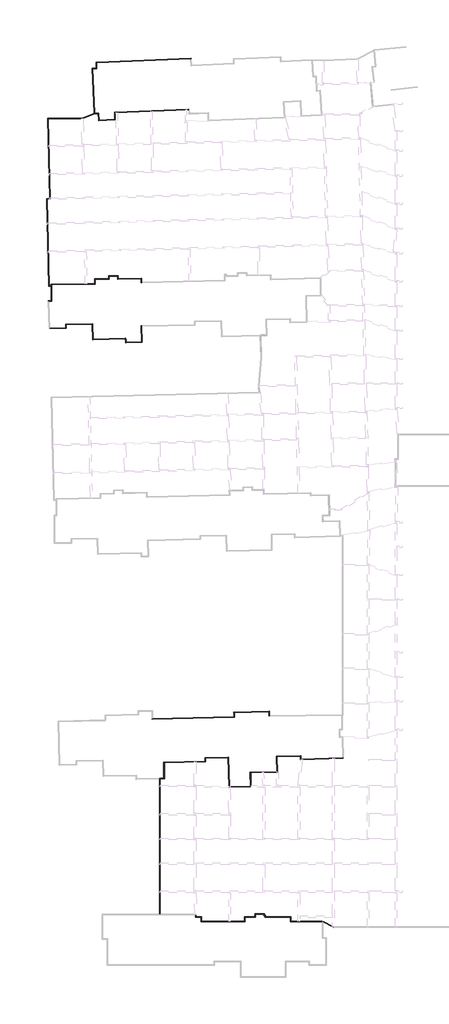
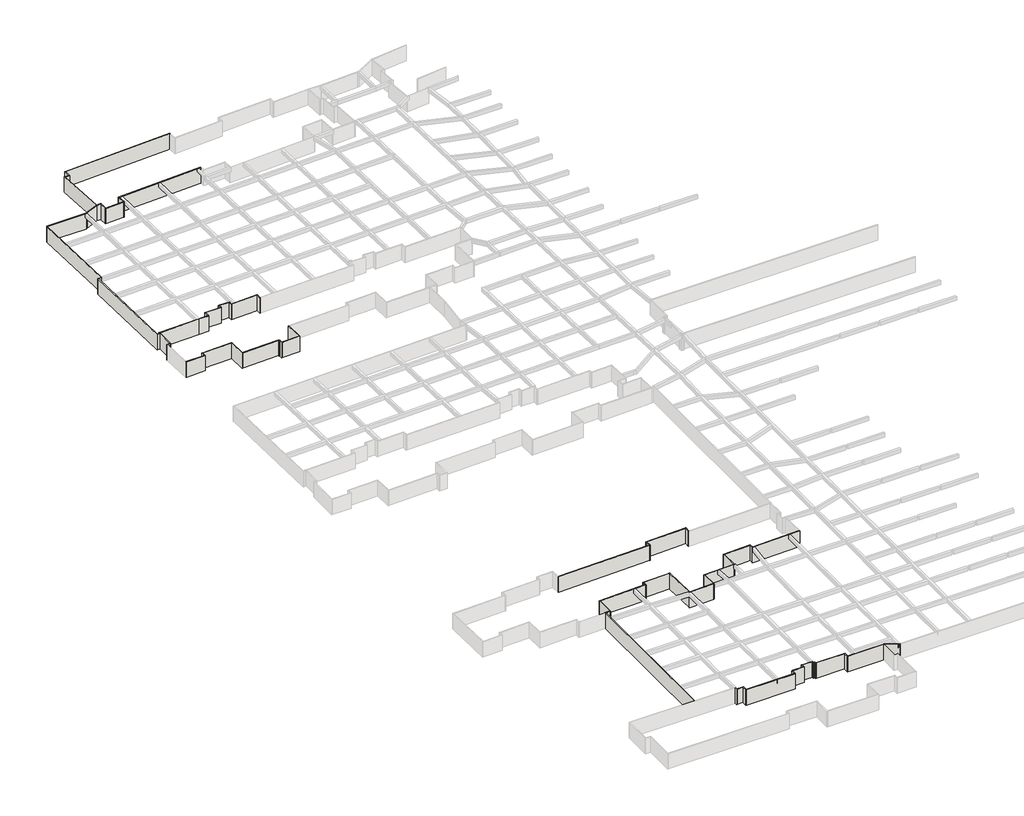
# One storey, part 2 of 20: 70 walls.
"""IFC4 building model written with IfcOpenShell, lengths in millimetres."""

import ifcopenshell
import ifcopenshell.guid

model = None  # the IFC model being written
_history = None  # IfcOwnerHistory: only IFC2X3 demands one
_inside = {}  # id of a spatial element -> (the spatial element, [elements in it])
_under = {}  # id of a project, library or spatial element -> (it, [spatial elements below it])
_declared = {}  # id of a project -> (the project, [libraries it declares])
_typed = {}  # id of a type object -> (the type object, [elements of that type])
_made_of = {}  # id of a material, layer set ... -> (it, [elements and type objects made of it])


def new_model(schema):
    """Start an empty IFC model of exactly this schema.

    Asked for "IFC4X3", IfcOpenShell would pick the latest addendum, in which some entities
    have other attributes; the version numbers below select the first issue.
    IFC2X3 requires an IfcOwnerHistory on every rooted entity: one is made here for all.
    """
    global model, _history
    if schema == "IFC4X3":
        model = ifcopenshell.file(schema_version=(4, 3, 0, 0))
    else:
        model = ifcopenshell.file(schema=schema)
    _inside.clear()
    _under.clear()
    _declared.clear()
    _typed.clear()
    _made_of.clear()
    _history = None
    if model.schema == "IFC2X3":
        org = make("IfcOrganization", Name="unknown")
        user = make(
            "IfcPersonAndOrganization",
            ThePerson=make("IfcPerson", FamilyName="unknown"),
            TheOrganization=org,
        )
        app = make(
            "IfcApplication",
            ApplicationDeveloper=org,
            Version="unknown",
            ApplicationFullName="unknown",
            ApplicationIdentifier="unknown",
        )
        _history = make(
            "IfcOwnerHistory",
            OwningUser=user,
            OwningApplication=app,
            ChangeAction="ADDED",
            CreationDate=0,
        )
    return model


def make(cls, **values):
    """One entity of the class cls with the attributes given. An attribute that is None is left unset."""
    return model.create_entity(
        cls, **{name: value for name, value in values.items() if value is not None}
    )


def rooted(cls, **values):
    """An entity with a GlobalId (a new one), such as an element, a storey or a relation."""
    return make(cls, GlobalId=ifcopenshell.guid.new(), OwnerHistory=_history, **values)


def si_unit(unit_type, name, prefix=None):
    """IfcSIUnit, for example si_unit("LENGTHUNIT", "METRE", prefix="MILLI")."""
    return make("IfcSIUnit", UnitType=unit_type, Prefix=prefix, Name=name)


def assignment(units):
    """IfcUnitAssignment: the units of a project."""
    return None if units is None else make("IfcUnitAssignment", Units=units)


def point(xyz):
    """IfcCartesianPoint."""
    return None if xyz is None else make("IfcCartesianPoint", Coordinates=xyz)


def direction(xyz):
    """IfcDirection."""
    return None if xyz is None else make("IfcDirection", DirectionRatios=xyz)


def frame(location, z_axis=None, x_axis=None):
    """IfcAxis2Placement3D, a coordinate frame: its origin and axes. An axis left out is left unset."""
    return make(
        "IfcAxis2Placement3D",
        Location=point(location),
        Axis=direction(z_axis),
        RefDirection=direction(x_axis),
    )


def origin():
    """The frame at (0, 0, 0) with its axes left unset."""
    return frame((0.0, 0.0, 0.0))


def origin_with_axes():
    """The frame at (0, 0, 0) with the z axis (0, 0, 1) and the x axis (1, 0, 0) written out."""
    return frame((0.0, 0.0, 0.0), z_axis=(0.0, 0.0, 1.0), x_axis=(1.0, 0.0, 0.0))


def place(relative_to, where):
    """IfcLocalPlacement: puts the frame where relative to a parent placement (None: the world)."""
    return make(
        "IfcLocalPlacement", PlacementRelTo=relative_to, RelativePlacement=where
    )


def context(
    kind, dimensions, precision=None, world=None, true_north=None, identifier=None
):
    """IfcGeometricRepresentationContext, for example the 3D "Model" context."""
    return make(
        "IfcGeometricRepresentationContext",
        ContextIdentifier=identifier,
        ContextType=kind,
        CoordinateSpaceDimension=dimensions,
        Precision=precision,
        WorldCoordinateSystem=world,
        TrueNorth=true_north,
    )


def project(units=None, contexts=None):
    """IfcProject with its units and contexts."""
    return rooted(
        "IfcProject",
        Name="project",
        RepresentationContexts=contexts,
        UnitsInContext=assignment(units),
    )


def spatial(cls, under=None, at=None, **own):
    """A site, building, storey or space (cls), placed at a placement, below another one or the project."""
    s = rooted(cls, ObjectPlacement=at, **own)
    if under is not None:
        _under.setdefault(under.id(), (under, []))[1].append(s)
    return s


def polyline(points):
    """IfcPolyline through the points."""
    return make("IfcPolyline", Points=[point(p) for p in points])


def outline(outer, holes=None, kind="AREA"):
    """IfcArbitraryClosedProfileDef: a profile drawn as a closed curve; with holes, ...WithVoids."""
    if holes is None:
        return make("IfcArbitraryClosedProfileDef", ProfileType=kind, OuterCurve=outer)
    return make(
        "IfcArbitraryProfileDefWithVoids",
        ProfileType=kind,
        OuterCurve=outer,
        InnerCurves=holes,
    )


def extrude(swept, where, along, depth):
    """IfcExtrudedAreaSolid: the profile swept, set in the frame where, extruded along a direction by depth."""
    return make(
        "IfcExtrudedAreaSolid",
        SweptArea=swept,
        Position=where,
        ExtrudedDirection=direction(along),
        Depth=depth,
    )


def faces_of(points, faces, orient=None, outer=None):
    """IfcFace entities. A face is a list of loops; a loop is a list of indices into points, from 0.

    orient and outer hold one flag for each loop. By default every Orientation is true, the
    first loop of a face is its IfcFaceOuterBound and the others are IfcFaceBound.
    """
    made = []
    for i, loops in enumerate(faces):
        bounds = []
        for j, loop in enumerate(loops):
            is_outer = j == 0 if outer is None else outer[i][j]
            bounds.append(
                make(
                    "IfcFaceOuterBound" if is_outer else "IfcFaceBound",
                    Bound=make("IfcPolyLoop", Polygon=[points[k] for k in loop]),
                    Orientation=True if orient is None else orient[i][j],
                )
            )
        made.append(make("IfcFace", Bounds=bounds))
    return made


def faceted_brep(points, faces, orient=None, outer=None, voids=None):
    """IfcFacetedBrep: a solid bounded by flat faces; with voids (closed shells), ...WithVoids."""
    shared = [point(p) for p in points]
    hull = make("IfcClosedShell", CfsFaces=faces_of(shared, faces, orient, outer))
    if voids is None:
        return make("IfcFacetedBrep", Outer=hull)
    return make(
        "IfcFacetedBrepWithVoids",
        Outer=hull,
        Voids=[
            make(cls, CfsFaces=faces_of(shared, fs, o, b)) for cls, fs, o, b in voids
        ],
    )


def shape(context_of_items, identifier, shape_type, items):
    """IfcShapeRepresentation: the items that make up one representation, for example the "Body"."""
    return make(
        "IfcShapeRepresentation",
        ContextOfItems=context_of_items,
        RepresentationIdentifier=identifier,
        RepresentationType=shape_type,
        Items=items,
    )


def made_of(thing, what):
    """Note that an element or type object is made of a material, layer set ...; save() writes the relation."""
    if what is not None:
        _made_of.setdefault(what.id(), (what, []))[1].append(thing)
    return thing


def element(
    cls,
    number,
    at=None,
    inside=None,
    cuts=None,
    type_object=None,
    material=None,
    context=None,
    identifier="Body",
    shape_type=None,
    held_by="IfcProductDefinitionShape",
    body=None,
    shapes=None,
    **own,
):
    """One element of the class cls, such as IfcWall. Its Tag is "e" and its number.

    at: its placement. inside: the storey or other place that contains it. cuts: it is an
    opening in that element (IfcRelVoidsElement). A single representation is given by context,
    identifier, shape_type and body (its items); several are given by shapes. held_by: the class
    of the entity that holds the representations. save() writes the other relations.
    """
    e = rooted(cls, Tag="e%d" % number, ObjectPlacement=at, **own)
    if body is not None:
        shapes = [shape(context, identifier, shape_type, body)]
    if shapes is not None:
        e.Representation = make(held_by, Representations=shapes)
    if inside is not None:
        _inside.setdefault(inside.id(), (inside, []))[1].append(e)
    if cuts is not None:
        rooted(
            "IfcRelVoidsElement", RelatingBuildingElement=cuts, RelatedOpeningElement=e
        )
    if type_object is not None:
        _typed.setdefault(type_object.id(), (type_object, []))[1].append(e)
    return made_of(e, material)


def aggregate(whole, parts):
    """IfcRelAggregates: a whole, such as a stair, and the parts it consists of."""
    return rooted("IfcRelAggregates", RelatingObject=whole, RelatedObjects=parts)


def save(model, path):
    """Write the relations noted so far, then the file.

    IfcRelAggregates (storeys below a building ...), IfcRelContainedInSpatialStructure (elements
    in a storey), IfcRelDefinesByType, IfcRelAssociatesMaterial and IfcRelDeclares: one each for
    every whole, place, type object, material and project.
    """
    for whole, parts in _under.values():
        aggregate(whole, parts)
    for where, things in _inside.values():
        rooted(
            "IfcRelContainedInSpatialStructure",
            RelatedElements=things,
            RelatingStructure=where,
        )
    for kind, things in _typed.values():
        rooted("IfcRelDefinesByType", RelatedObjects=things, RelatingType=kind)
    for what, things in _made_of.values():
        rooted("IfcRelAssociatesMaterial", RelatedObjects=things, RelatingMaterial=what)
    for by, libraries in _declared.values():
        rooted("IfcRelDeclares", RelatingContext=by, RelatedDefinitions=libraries)
    model.write(path)


model = new_model("IFC4")

# Units and contexts
model_context = context("Model", 3, world=origin())
ifc_project = project(units=[si_unit("LENGTHUNIT", "METRE", prefix="MILLI")], contexts=[model_context])

# Site, building, storey
site = spatial("IfcSite", under=ifc_project)
building = spatial("IfcBuilding", under=site)
storey = spatial("IfcBuildingStorey", under=building, Name="户型图", Elevation=0.0)

# Walls
placement = place(None, origin())
element("IfcWall", 1, ObjectType="所有墙体", at=placement, inside=storey, context=model_context, shape_type="Brep", body=[
    faceted_brep([(-25950.6212592, 186690.2553865, 0.0), (-25511.4176052, 168328.5480808, 0.0), (-25508.5480808, 168208.5823948, 0.0), (-25508.5480808, 168208.5823948, 3300.0), (-25511.4176052, 168328.5480808, 3300.0), (-25950.6212592, 186690.2553865, 3300.0), (-25830.5869354, 186690.2553865, 0.0), (-25830.5869354, 186690.2553865, 3300.0), (-25388.5823948, 168211.4519192, 3300.0), (-25388.5823948, 168211.4519192, 0.0)], [[[0, 1, 2, 3, 4, 5]], [[6, 7, 8, 9]], [[2, 1, 0, 6, 9]], [[5, 4, 3, 8, 7]], [[3, 2, 9, 8]], [[0, 5, 7, 6]]]),
])
element("IfcWall", 2, ObjectType="所有墙体", at=placement, inside=storey, context=model_context, shape_type="Brep", body=[
    faceted_brep([(-25511.4176052, 168328.5480808, 0.0), (-26211.4966602, 168311.8025095, 0.0), (-26211.4966602, 168311.8025095, 3300.0), (-25511.4176052, 168328.5480808, 3300.0), (-25508.5480808, 168208.5823948, 0.0), (-25508.5480808, 168208.5823948, 3300.0), (-26088.6614497, 168194.7063479, 3300.0), (-26208.6271358, 168191.8368235, 3300.0), (-26208.6271358, 168191.8368235, 0.0), (-26088.6614497, 168194.7063479, 0.0)], [[[0, 1, 2, 3]], [[4, 5, 6, 7, 8, 9]], [[1, 0, 4, 9, 8]], [[3, 2, 7, 6, 5]], [[0, 3, 5, 4]], [[2, 1, 8, 7]]]),
])
element("IfcWall", 3, ObjectType="所有墙体", at=placement, inside=storey, context=model_context, shape_type="Brep", body=[
    faceted_brep([(-26208.6271358, 168191.8368235, 0.0), (-25728.0157025, 148099.0020152, 0.0), (-25728.0157025, 148099.0020152, 3300.0), (-26208.6271358, 168191.8368235, 3300.0), (-26088.6614497, 168194.7063479, 0.0), (-26088.6614497, 168194.7063479, 3300.0), (-25610.8517239, 148219.0020152, 3300.0), (-25607.9813787, 148099.0020152, 3300.0), (-25607.9813787, 148099.0020152, 0.0), (-25610.8517239, 148219.0020152, 0.0)], [[[0, 1, 2, 3]], [[4, 5, 6, 7, 8, 9]], [[1, 0, 4, 9, 8]], [[3, 2, 7, 6, 5]], [[0, 3, 5, 4]], [[2, 1, 8, 7]]]),
])
element("IfcWall", 4, ObjectType="所有墙体", at=placement, inside=storey, context=model_context, shape_type="SweptSolid", body=[
    extrude(outline(polyline([(-25178.2753849, 148099.0020152), (-25607.9813787, 148099.0020152), (-25610.8517239, 148219.0020152), (-25178.2753849, 148219.0020152), (-25178.2753849, 148099.0020152)])), origin_with_axes(), (0.0, 0.0, 1.0), 3300.0),
])
element("IfcWall", 5, ObjectType="所有墙体", at=placement, inside=storey, context=model_context, shape_type="Brep", body=[
    faceted_brep([(-25129.4337132, 148099.0020152, 0.0), (-25129.4337132, 144672.0423241, 0.0), (-25129.4337132, 144552.0423241, 0.0), (-25129.4337132, 144552.0423241, 3300.0), (-25129.4337132, 144672.0423241, 3300.0), (-25129.4337132, 148099.0020152, 3300.0), (-25009.4337132, 148099.0020152, 0.0), (-25009.4337132, 148099.0020152, 3300.0), (-25009.4337132, 144552.0423241, 3300.0), (-25009.4337132, 144552.0423241, 0.0), (-25058.2753849, 148099.0020152, 0.0), (-25058.2753849, 148099.0020152, 3300.0)], [[[0, 1, 2, 3, 4, 5]], [[6, 7, 8, 9]], [[2, 1, 0, 10, 6, 9]], [[5, 4, 3, 8, 7, 11]], [[3, 2, 9, 8]], [[0, 5, 11, 7, 6, 10]]]),
])
element("IfcWall", 6, ObjectType="所有墙体", at=placement, inside=storey, context=model_context, shape_type="Brep", body=[
    faceted_brep([(-25129.4337132, 144672.0423241, 0.0), (-25791.8650311, 144672.0423241, 0.0), (-25791.8650311, 144672.0423241, 3300.0), (-25129.4337132, 144672.0423241, 3300.0), (-25129.4337132, 144552.0423241, 0.0), (-25129.4337132, 144552.0423241, 3300.0), (-25668.9144149, 144552.0423241, 3300.0), (-25788.9498199, 144552.0423241, 3300.0), (-25788.9498199, 144552.0423241, 0.0), (-25668.9144149, 144552.0423241, 0.0)], [[[0, 1, 2, 3]], [[4, 5, 6, 7, 8, 9]], [[1, 0, 4, 9, 8]], [[3, 2, 7, 6, 5]], [[0, 3, 5, 4]], [[2, 1, 8, 7]]]),
])
element("IfcWall", 7, ObjectType="所有墙体", at=placement, inside=storey, context=model_context, shape_type="Brep", body=[
    faceted_brep([(-25515.5605216, 138239.4748729, 0.0), (-21616.5538771, 138334.1951042, 0.0), (-21616.5538771, 138334.1951042, 3300.0), (-25515.5605216, 138239.4748729, 3300.0), (-25518.4748729, 138359.4394784, 0.0), (-25518.4748729, 138359.4394784, 3300.0), (-21739.4328339, 138451.2453583, 3300.0), (-21619.4682284, 138454.1597097, 3300.0), (-21619.4682284, 138454.1597097, 0.0), (-21739.4328339, 138451.2453583, 0.0)], [[[0, 1, 2, 3]], [[4, 5, 6, 7, 8, 9]], [[1, 0, 4, 9, 8]], [[3, 2, 7, 6, 5]], [[0, 3, 5, 4]], [[2, 1, 8, 7]]]),
])
element("IfcWall", 8, ObjectType="所有墙体", at=placement, inside=storey, context=model_context, shape_type="Brep", body=[
    faceted_brep([(-21619.4682284, 138454.1597097, 0.0), (-21635.9951586, 139134.4643242, 0.0), (-21638.9095099, 139254.4289296, 0.0), (-21638.9095099, 139254.4289296, 3300.0), (-21635.9951586, 139134.4643242, 3300.0), (-21619.4682284, 138454.1597097, 3300.0), (-21739.4328339, 138451.2453583, 0.0), (-21739.4328339, 138451.2453583, 3300.0), (-21758.8741153, 139251.5145783, 3300.0), (-21758.8741153, 139251.5145783, 0.0)], [[[0, 1, 2, 3, 4, 5]], [[6, 7, 8, 9]], [[2, 1, 0, 6, 9]], [[5, 4, 3, 8, 7]], [[0, 5, 7, 6]], [[3, 2, 9, 8]]]),
])
element("IfcWall", 9, ObjectType="所有墙体", at=placement, inside=storey, context=model_context, shape_type="Brep", body=[
    faceted_brep([(-21635.9951586, 139134.4643242, 0.0), (-15657.5285806, 139279.7017625, 0.0), (-15537.5639751, 139282.6161138, 0.0), (-15537.5639751, 139282.6161138, 3300.0), (-15657.5285806, 139279.7017625, 3300.0), (-21635.9951586, 139134.4643242, 3300.0), (-21638.9095099, 139254.4289296, 0.0), (-21638.9095099, 139254.4289296, 3300.0), (-15540.4783265, 139402.5807193, 3300.0), (-15540.4783265, 139402.5807193, 0.0)], [[[0, 1, 2, 3, 4, 5]], [[6, 7, 8, 9]], [[2, 1, 0, 6, 9]], [[5, 4, 3, 8, 7]], [[0, 5, 7, 6]], [[3, 2, 9, 8]]]),
])
element("IfcWall", 10, ObjectType="所有墙体", at=placement, inside=storey, context=model_context, shape_type="Brep", body=[
    faceted_brep([(-15657.5285806, 139279.7017625, 0.0), (-15570.0927706, 135680.5466563, 0.0), (-15570.0927706, 135680.5466563, 3300.0), (-15657.5285806, 139279.7017625, 3300.0), (-15537.5639751, 139282.6161138, 0.0), (-15537.5639751, 139282.6161138, 3300.0), (-15453.0425165, 135803.4256131, 3300.0), (-15450.1281652, 135683.4610077, 3300.0), (-15450.1281652, 135683.4610077, 0.0), (-15453.0425165, 135803.4256131, 0.0)], [[[0, 1, 2, 3]], [[4, 5, 6, 7, 8, 9]], [[1, 0, 4, 9, 8]], [[3, 2, 7, 6, 5]], [[0, 3, 5, 4]], [[2, 1, 8, 7]]]),
])
element("IfcWall", 11, ObjectType="所有墙体", at=placement, inside=storey, context=model_context, shape_type="SweptSolid", body=[
    extrude(outline(polyline([(-8078.975172, 135862.531571), (-15450.1281652, 135683.4610077), (-15453.0425165, 135803.4256131), (-8078.975172, 135982.566976), (-8078.975172, 135862.531571)])), origin_with_axes(), (0.0, 0.0, 1.0), 3300.0),
])
element("IfcWall", 12, ObjectType="所有墙体", at=placement, inside=storey, context=model_context, shape_type="Brep", body=[
    faceted_brep([(-8078.975172, 135982.566976, 0.0), (-8078.975172, 135862.531571, 0.0), (-8078.975172, 135664.0068791, 0.0), (-8078.975172, 135664.0068791, 3300.0), (-8078.975172, 135862.531571, 3300.0), (-8078.975172, 135982.566976, 3300.0), (-7958.975172, 135985.4821872, 0.0), (-7958.975172, 135985.4821872, 3300.0), (-7958.975172, 135784.0068791, 3300.0), (-7958.975172, 135664.0068791, 3300.0), (-7958.975172, 135664.0068791, 0.0), (-7958.975172, 135784.0068791, 0.0)], [[[0, 1, 2, 3, 4, 5]], [[6, 7, 8, 9, 10, 11]], [[2, 1, 0, 6, 11, 10]], [[5, 4, 3, 9, 8, 7]], [[0, 5, 7, 6]], [[3, 2, 10, 9]]]),
])
element("IfcWall", 13, ObjectType="所有墙体", at=placement, inside=storey, context=model_context, shape_type="Brep", body=[
    faceted_brep([(-7958.975172, 135664.0068791, 0.0), (-7918.9028855, 135664.0068791, 0.0), (-7798.9028855, 135664.0068791, 0.0), (-7798.9028855, 135664.0068791, 3300.0), (-7918.9028855, 135664.0068791, 3300.0), (-7958.975172, 135664.0068791, 3300.0), (-7958.975172, 135784.0068791, 0.0), (-7958.975172, 135784.0068791, 3300.0), (-7798.9028855, 135784.0068791, 3300.0), (-7798.9028855, 135784.0068791, 0.0)], [[[0, 1, 2, 3, 4, 5]], [[6, 7, 8, 9]], [[2, 1, 0, 6, 9]], [[5, 4, 3, 8, 7]], [[0, 5, 7, 6]], [[3, 2, 9, 8]]]),
])
element("IfcWall", 14, ObjectType="所有墙体", at=placement, inside=storey, context=model_context, shape_type="Brep", body=[
    faceted_brep([(-7918.9028855, 135664.0068791, 0.0), (-7918.9028855, 134967.1170586, 0.0), (-7918.9028855, 134967.1170586, 3300.0), (-7918.9028855, 135664.0068791, 3300.0), (-7798.9028855, 135664.0068791, 0.0), (-7798.9028855, 135664.0068791, 3300.0), (-7798.9028855, 135090.0676748, 3300.0), (-7798.9028855, 134970.0322698, 3300.0), (-7798.9028855, 134970.0322698, 0.0), (-7798.9028855, 135090.0676748, 0.0)], [[[0, 1, 2, 3]], [[4, 5, 6, 7, 8, 9]], [[1, 0, 4, 9, 8]], [[3, 2, 7, 6, 5]], [[0, 3, 5, 4]], [[2, 1, 8, 7]]]),
])
element("IfcWall", 15, ObjectType="所有墙体", at=placement, inside=storey, context=model_context, shape_type="Brep", body=[
    faceted_brep([(-7798.9028855, 134970.0322698, 0.0), (-4138.5429414, 135058.954955, 0.0), (-4138.5429414, 135058.954955, 3300.0), (-7798.9028855, 134970.0322698, 3300.0), (-7798.9028855, 135090.0676748, 0.0), (-7798.9028855, 135090.0676748, 3300.0), (-4261.4218982, 135176.0052091, 3300.0), (-4141.4572928, 135178.9195604, 3300.0), (-4141.4572928, 135178.9195604, 0.0), (-4261.4218982, 135176.0052091, 0.0)], [[[0, 1, 2, 3]], [[4, 5, 6, 7, 8, 9]], [[1, 0, 4, 9, 8]], [[3, 2, 7, 6, 5]], [[0, 3, 5, 4]], [[2, 1, 8, 7]]]),
])
element("IfcWall", 16, ObjectType="所有墙体", at=placement, inside=storey, context=model_context, shape_type="Brep", body=[
    faceted_brep([(-4141.4572928, 135178.9195604, 0.0), (-4228.4021072, 138757.8636225, 0.0), (-4231.3164585, 138877.8282279, 0.0), (-4231.3164585, 138877.8282279, 3300.0), (-4228.4021072, 138757.8636225, 3300.0), (-4141.4572928, 135178.9195604, 3300.0), (-4261.4218982, 135176.0052091, 0.0), (-4261.4218982, 135176.0052091, 3300.0), (-4351.281064, 138874.9138766, 3300.0), (-4351.281064, 138874.9138766, 0.0)], [[[0, 1, 2, 3, 4, 5]], [[6, 7, 8, 9]], [[2, 1, 0, 6, 9]], [[5, 4, 3, 8, 7]], [[0, 5, 7, 6]], [[3, 2, 9, 8]]]),
])
element("IfcWall", 17, ObjectType="所有墙体", at=placement, inside=storey, context=model_context, shape_type="Brep", body=[
    faceted_brep([(25412.5739519, 48794.2395474, 0.0), (25412.5739519, 49895.3149226, 0.0), (25412.5739519, 49895.3149226, 3300.0), (25412.5739519, 48794.2395474, 3300.0), (25292.5739519, 48792.1449396, 0.0), (25292.5739519, 48792.1449396, 3300.0), (25292.5739519, 49771.051285, 3300.0), (25292.5739519, 49891.1244303, 3300.0), (25292.5739519, 49891.1244303, 0.0), (25292.5739519, 49771.051285, 0.0)], [[[0, 1, 2, 3]], [[4, 5, 6, 7, 8, 9]], [[1, 0, 4, 9, 8]], [[3, 2, 7, 6, 5]], [[0, 3, 5, 4]], [[2, 1, 8, 7]]]),
])
element("IfcWall", 18, ObjectType="所有墙体", at=placement, inside=storey, context=model_context, shape_type="Brep", body=[
    faceted_brep([(25292.5739519, 49891.1244303, 0.0), (17095.5117509, 49604.8767107, 0.0), (17095.5117509, 49604.8767107, 3300.0), (25292.5739519, 49891.1244303, 3300.0), (25292.5739519, 49771.051285, 0.0), (25292.5739519, 49771.051285, 3300.0), (17219.6265897, 49489.137751, 3300.0), (17099.6996905, 49484.9498114, 3300.0), (17099.6996905, 49484.9498114, 0.0), (17219.6265897, 49489.137751, 0.0)], [[[0, 1, 2, 3]], [[4, 5, 6, 7, 8, 9]], [[1, 0, 4, 9, 8]], [[3, 2, 7, 6, 5]], [[0, 3, 5, 4]], [[2, 1, 8, 7]]]),
])
element("IfcWall", 19, ObjectType="所有墙体", at=placement, inside=storey, context=model_context, shape_type="Brep", body=[
    faceted_brep([(17099.6996905, 49484.9498114, 0.0), (17132.2770227, 48552.0570742, 0.0), (17136.4652061, 48432.123195, 0.0), (17136.4652061, 48432.123195, 3300.0), (17132.2770227, 48552.0570742, 3300.0), (17099.6996905, 49484.9498114, 3300.0), (17219.6265897, 49489.137751, 0.0), (17219.6265897, 49489.137751, 3300.0), (17256.4372899, 48435.0172167, 3300.0), (17256.4372899, 48435.0172167, 0.0)], [[[0, 1, 2, 3, 4, 5]], [[6, 7, 8, 9]], [[2, 1, 0, 6, 9]], [[5, 4, 3, 8, 7]], [[0, 5, 7, 6]], [[3, 2, 9, 8]]]),
])
element("IfcWall", 20, ObjectType="所有墙体", at=placement, inside=storey, context=model_context, shape_type="Brep", body=[
    faceted_brep([(17132.2770227, 48552.0570742, 0.0), (-1631.4643758, 48099.4294775, 0.0), (-1751.4294775, 48096.5356242, 0.0), (-1751.4294775, 48096.5356242, 3300.0), (-1631.4643758, 48099.4294775, 3300.0), (17132.2770227, 48552.0570742, 3300.0), (17136.4652061, 48432.123195, 0.0), (17136.4652061, 48432.123195, 3300.0), (-1748.5356242, 47976.5705225, 3300.0), (-1748.5356242, 47976.5705225, 0.0)], [[[0, 1, 2, 3, 4, 5]], [[6, 7, 8, 9]], [[2, 1, 0, 6, 9]], [[5, 4, 3, 8, 7]], [[0, 5, 7, 6]], [[3, 2, 9, 8]]]),
])
element("IfcWall", 21, ObjectType="所有墙体", at=placement, inside=storey, context=model_context, shape_type="SweptSolid", body=[
    extrude(outline(polyline([(-39.60639, 2935.916483), (-39.60639, 34214.4516812), (80.39361, 34217.3463764), (80.39361, 2935.916483), (-39.60639, 2935.916483)])), origin_with_axes(), (0.0, 0.0, 1.0), 3300.0),
])
element("IfcWall", 22, ObjectType="所有墙体", at=placement, inside=storey, context=model_context, shape_type="Brep", body=[
    faceted_brep([(37775.0, 1211.1432311, 0.0), (40172.2935798, -63.5203758, 0.0), (40172.2935798, -63.5203758, 3300.0), (37775.0, 1211.1432311, 3300.0), (37775.0, 1347.0516371, 0.0), (37775.0, 1347.0516371, 3300.0), (40202.2129402, 56.4796242, 3300.0), (40427.900116, -63.5203758, 3300.0), (40427.900116, -63.5203758, 0.0), (40202.2129402, 56.4796242, 0.0)], [[[0, 1, 2, 3]], [[4, 5, 6, 7, 8, 9]], [[1, 0, 4, 9, 8]], [[3, 2, 7, 6, 5]], [[0, 3, 5, 4]], [[2, 1, 8, 7]]]),
])
element("IfcWall", 23, ObjectType="所有墙体", at=placement, inside=storey, context=model_context, shape_type="Brep", body=[
    faceted_brep([(6671.8561293, 188959.2892299, 0.0), (-10511.0814854, 188193.3552038, 0.0), (-10511.0814854, 188193.3552038, 3300.0), (6671.8561293, 188959.2892299, 3300.0), (6677.199855, 188839.4082698, 0.0), (6677.199855, 188839.4082698, 3300.0), (-10385.8567995, 188078.8179695, 3300.0), (-10505.7377596, 188073.4742437, 3300.0), (-10505.7377596, 188073.4742437, 0.0), (-10385.8567995, 188078.8179695, 0.0)], [[[0, 1, 2, 3]], [[4, 5, 6, 7, 8, 9]], [[1, 0, 4, 9, 8]], [[3, 2, 7, 6, 5]], [[0, 3, 5, 4]], [[2, 1, 8, 7]]]),
])
element("IfcWall", 24, ObjectType="所有墙体", at=placement, inside=storey, context=model_context, shape_type="Brep", body=[
    faceted_brep([(-10505.7377596, 188073.4742437, 0.0), (-10439.736954, 186592.8144393, 0.0), (-10434.3932282, 186472.9334792, 0.0), (-10434.3932282, 186472.9334792, 3300.0), (-10439.736954, 186592.8144393, 3300.0), (-10505.7377596, 188073.4742437, 3300.0), (-10385.8567995, 188078.8179695, 0.0), (-10385.8567995, 188078.8179695, 3300.0), (-10314.5122681, 186478.2772049, 3300.0), (-10314.5122681, 186478.2772049, 0.0)], [[[0, 1, 2, 3, 4, 5]], [[6, 7, 8, 9]], [[2, 1, 0, 6, 9]], [[5, 4, 3, 8, 7]], [[0, 5, 7, 6]], [[3, 2, 9, 8]]]),
])
element("IfcWall", 25, ObjectType="所有墙体", at=placement, inside=storey, context=model_context, shape_type="Brep", body=[
    faceted_brep([(-10439.736954, 186592.8144393, 0.0), (-14060.7215407, 186431.4080858, 0.0), (-14180.6025008, 186426.06436, 0.0), (-14180.6025008, 186426.06436, 3300.0), (-14060.7215407, 186431.4080858, 3300.0), (-10439.736954, 186592.8144393, 3300.0), (-10434.3932282, 186472.9334792, 0.0), (-10434.3932282, 186472.9334792, 3300.0), (-14175.258775, 186306.1833999, 3300.0), (-14175.258775, 186306.1833999, 0.0)], [[[0, 1, 2, 3, 4, 5]], [[6, 7, 8, 9]], [[2, 1, 0, 6, 9]], [[5, 4, 3, 8, 7]], [[0, 5, 7, 6]], [[3, 2, 9, 8]]]),
])
element("IfcWall", 26, ObjectType="所有墙体", at=placement, inside=storey, context=model_context, shape_type="Brep", body=[
    faceted_brep([(-14060.7215407, 186431.4080858, 0.0), (-14131.9496261, 188029.3365074, 0.0), (-14131.9496261, 188029.3365074, 3300.0), (-14060.7215407, 186431.4080858, 3300.0), (-14180.6025008, 186426.06436, 0.0), (-14180.6025008, 186426.06436, 3300.0), (-14246.7197522, 187909.3365074, 3300.0), (-14252.0687842, 188029.3365074, 3300.0), (-14252.0687842, 188029.3365074, 0.0), (-14246.7197522, 187909.3365074, 0.0)], [[[0, 1, 2, 3]], [[4, 5, 6, 7, 8, 9]], [[1, 0, 4, 9, 8]], [[3, 2, 7, 6, 5]], [[0, 3, 5, 4]], [[2, 1, 8, 7]]]),
])
element("IfcWall", 27, ObjectType="所有墙体", at=placement, inside=storey, context=model_context, shape_type="Brep", body=[
    faceted_brep([(-14252.0687842, 188029.3365074, 0.0), (-15101.5418272, 188029.3365074, 0.0), (-15101.5418272, 188029.3365074, 3300.0), (-14252.0687842, 188029.3365074, 3300.0), (-14246.7197522, 187909.3365074, 0.0), (-14246.7197522, 187909.3365074, 3300.0), (-15077.1275512, 187909.3365074, 3300.0), (-15384.2441111, 187909.3365074, 3300.0), (-15384.2441111, 187909.3365074, 0.0), (-15077.1275512, 187909.3365074, 0.0)], [[[0, 1, 2, 3]], [[4, 5, 6, 7, 8, 9]], [[1, 0, 4, 9, 8]], [[3, 2, 7, 6, 5]], [[0, 3, 5, 4]], [[2, 1, 8, 7]]]),
])
element("IfcWall", 28, ObjectType="所有墙体", at=placement, inside=storey, context=model_context, shape_type="SweptSolid", body=[
    extrude(outline(polyline([(-17973.5169699, 186810.2553865), (-15384.2441111, 187909.3365074), (-15077.1275512, 187909.3365074), (-17666.4004101, 186810.2553865), (-17973.5169699, 186810.2553865)])), origin_with_axes(), (0.0, 0.0, 1.0), 3300.0),
])
element("IfcWall", 29, ObjectType="所有墙体", at=placement, inside=storey, context=model_context, shape_type="Brep", body=[
    faceted_brep([(-17666.4004101, 186810.2553865, 0.0), (-25953.4916044, 186810.2553865, 0.0), (-25953.4916044, 186810.2553865, 3300.0), (-17666.4004101, 186810.2553865, 3300.0), (-17949.102694, 186690.2553865, 0.0), (-17949.102694, 186690.2553865, 3300.0), (-25830.5869354, 186690.2553865, 3300.0), (-25950.6212592, 186690.2553865, 3300.0), (-25950.6212592, 186690.2553865, 0.0), (-25830.5869354, 186690.2553865, 0.0)], [[[0, 1, 2, 3]], [[4, 5, 6, 7, 8, 9]], [[1, 0, 4, 9, 8]], [[3, 2, 7, 6, 5]], [[2, 1, 8, 7]], [[0, 3, 5, 4]]]),
])
element("IfcWall", 30, ObjectType="所有墙体", at=placement, inside=storey, context=model_context, shape_type="Brep", body=[
    faceted_brep([(-15031.9496261, 188029.3365074, 0.0), (-15489.7234937, 198299.0197162, 0.0), (-15495.0725257, 198419.0197162, 0.0), (-15495.0725257, 198419.0197162, 3300.0), (-15489.7234937, 198299.0197162, 3300.0), (-15031.9496261, 188029.3365074, 3300.0), (-15151.1305129, 188008.2873591, 0.0), (-15151.1305129, 188008.2873591, 3300.0), (-15615.1916838, 198419.0197162, 3300.0), (-15615.1916838, 198419.0197162, 0.0), (-15101.5418272, 188029.3365074, 0.0), (-15101.5418272, 188029.3365074, 3300.0)], [[[0, 1, 2, 3, 4, 5]], [[6, 7, 8, 9]], [[2, 1, 0, 10, 6, 9]], [[5, 4, 3, 8, 7, 11]], [[3, 2, 9, 8]], [[0, 5, 11, 10]], [[11, 7, 6, 10]]]),
])
element("IfcWall", 31, ObjectType="所有墙体", at=placement, inside=storey, context=model_context, shape_type="Brep", body=[
    faceted_brep([(-15489.7234937, 198299.0197162, 0.0), (-14589.7234937, 198299.0197162, 0.0), (-14589.7234937, 198299.0197162, 3300.0), (-15489.7234937, 198299.0197162, 3300.0), (-15495.0725257, 198419.0197162, 0.0), (-15495.0725257, 198419.0197162, 3300.0), (-14715.1916838, 198419.0197162, 3300.0), (-14595.0725257, 198419.0197162, 3300.0), (-14595.0725257, 198419.0197162, 0.0), (-14715.1916838, 198419.0197162, 0.0)], [[[0, 1, 2, 3]], [[4, 5, 6, 7, 8, 9]], [[1, 0, 4, 9, 8]], [[3, 2, 7, 6, 5]], [[0, 3, 5, 4]], [[2, 1, 8, 7]]]),
])
element("IfcWall", 32, ObjectType="所有墙体", at=placement, inside=storey, context=model_context, shape_type="Brep", body=[
    faceted_brep([(-14595.0725257, 198419.0197162, 0.0), (-14649.8663989, 199648.2635852, 0.0), (-14655.2101247, 199768.1445453, 0.0), (-14655.2101247, 199768.1445453, 3300.0), (-14649.8663989, 199648.2635852, 3300.0), (-14595.0725257, 198419.0197162, 3300.0), (-14715.1916838, 198419.0197162, 0.0), (-14715.1916838, 198419.0197162, 3300.0), (-14775.0910848, 199762.8008196, 3300.0), (-14775.0910848, 199762.8008196, 0.0)], [[[0, 1, 2, 3, 4, 5]], [[6, 7, 8, 9]], [[2, 1, 0, 6, 9]], [[5, 4, 3, 8, 7]], [[0, 5, 7, 6]], [[3, 2, 9, 8]]]),
])
element("IfcWall", 33, ObjectType="所有墙体", at=placement, inside=storey, context=model_context, shape_type="Brep", body=[
    faceted_brep([(-14649.8663989, 199648.2635852, 0.0), (7101.7994998, 200617.8498929, 0.0), (7221.6804599, 200623.1936187, 0.0), (7221.6804599, 200623.1936187, 3300.0), (7101.7994998, 200617.8498929, 3300.0), (-14649.8663989, 199648.2635852, 3300.0), (-14655.2101247, 199768.1445453, 0.0), (-14655.2101247, 199768.1445453, 3300.0), (7216.3367341, 200743.0745788, 3300.0), (7216.3367341, 200743.0745788, 0.0)], [[[0, 1, 2, 3, 4, 5]], [[6, 7, 8, 9]], [[2, 1, 0, 6, 9]], [[5, 4, 3, 8, 7]], [[0, 5, 7, 6]], [[3, 2, 9, 8]]]),
])
element("IfcWall", 34, ObjectType="所有墙体", at=placement, inside=storey, context=model_context, shape_type="Brep", body=[
    faceted_brep([(8257.0, 2815.916483, 0.0), (8257.0, 2250.0, 0.0), (8257.0, 2250.0, 3300.0), (8257.0, 2815.916483, 3300.0), (8377.0, 2815.916483, 0.0), (8377.0, 2815.916483, 3300.0), (8377.0, 2370.0, 3300.0), (8377.0, 2250.0, 3300.0), (8377.0, 2250.0, 0.0), (8377.0, 2370.0, 0.0)], [[[0, 1, 2, 3]], [[4, 5, 6, 7, 8, 9]], [[1, 0, 4, 9, 8]], [[3, 2, 7, 6, 5]], [[0, 3, 5, 4]], [[2, 1, 8, 7]]]),
])
element("IfcWall", 35, ObjectType="所有墙体", at=placement, inside=storey, context=model_context, shape_type="Brep", body=[
    faceted_brep([(8377.0, 2250.0, 0.0), (9557.0, 2250.0, 0.0), (9677.0, 2250.0, 0.0), (9677.0, 2250.0, 3300.0), (9557.0, 2250.0, 3300.0), (8377.0, 2250.0, 3300.0), (8377.0, 2370.0, 0.0), (8377.0, 2370.0, 3300.0), (9677.0, 2370.0, 3300.0), (9677.0, 2370.0, 0.0)], [[[0, 1, 2, 3, 4, 5]], [[6, 7, 8, 9]], [[2, 1, 0, 6, 9]], [[5, 4, 3, 8, 7]], [[0, 5, 7, 6]], [[3, 2, 9, 8]]]),
])
element("IfcWall", 36, ObjectType="所有墙体", at=placement, inside=storey, context=model_context, shape_type="Brep", body=[
    faceted_brep([(9557.0, 2250.0, 0.0), (9557.0, 1251.0, 0.0), (9557.0, 1251.0, 3300.0), (9557.0, 2250.0, 3300.0), (9677.0, 2250.0, 0.0), (9677.0, 2250.0, 3300.0), (9677.0, 1371.0, 3300.0), (9677.0, 1251.0, 3300.0), (9677.0, 1251.0, 0.0), (9677.0, 1371.0, 0.0)], [[[0, 1, 2, 3]], [[4, 5, 6, 7, 8, 9]], [[1, 0, 4, 9, 8]], [[3, 2, 7, 6, 5]], [[0, 3, 5, 4]], [[2, 1, 8, 7]]]),
])
element("IfcWall", 37, ObjectType="所有墙体", at=placement, inside=storey, context=model_context, shape_type="Brep", body=[
    faceted_brep([(9677.0, 1251.0, 0.0), (19676.0, 1251.0, 0.0), (19676.0, 1251.0, 3300.0), (9677.0, 1251.0, 3300.0), (9677.0, 1371.0, 0.0), (9677.0, 1371.0, 3300.0), (19556.0, 1371.0, 3300.0), (19676.0, 1371.0, 3300.0), (19676.0, 1371.0, 0.0), (19556.0, 1371.0, 0.0)], [[[0, 1, 2, 3]], [[4, 5, 6, 7, 8, 9]], [[1, 0, 4, 9, 8]], [[3, 2, 7, 6, 5]], [[0, 3, 5, 4]], [[2, 1, 8, 7]]]),
])
element("IfcWall", 38, ObjectType="所有墙体", at=placement, inside=storey, context=model_context, shape_type="Brep", body=[
    faceted_brep([(19676.0, 1371.0, 0.0), (19676.0, 2250.0, 0.0), (19676.0, 2370.0, 0.0), (19676.0, 2370.0, 3300.0), (19676.0, 2250.0, 3300.0), (19676.0, 1371.0, 3300.0), (19556.0, 1371.0, 0.0), (19556.0, 1371.0, 3300.0), (19556.0, 2370.0, 3300.0), (19556.0, 2370.0, 0.0)], [[[0, 1, 2, 3, 4, 5]], [[6, 7, 8, 9]], [[2, 1, 0, 6, 9]], [[5, 4, 3, 8, 7]], [[0, 5, 7, 6]], [[3, 2, 9, 8]]]),
])
element("IfcWall", 39, ObjectType="所有墙体", at=placement, inside=storey, context=model_context, shape_type="Brep", body=[
    faceted_brep([(19676.0, 2250.0, 0.0), (22076.0, 2250.0, 0.0), (22076.0, 2250.0, 3300.0), (19676.0, 2250.0, 3300.0), (19676.0, 2370.0, 0.0), (19676.0, 2370.0, 3300.0), (21956.0, 2370.0, 3300.0), (22076.0, 2370.0, 3300.0), (22076.0, 2370.0, 0.0), (21956.0, 2370.0, 0.0)], [[[0, 1, 2, 3]], [[4, 5, 6, 7, 8, 9]], [[1, 0, 4, 9, 8]], [[3, 2, 7, 6, 5]], [[0, 3, 5, 4]], [[2, 1, 8, 7]]]),
])
element("IfcWall", 40, ObjectType="所有墙体", at=placement, inside=storey, context=model_context, shape_type="Brep", body=[
    faceted_brep([(22076.0, 2370.0, 0.0), (22076.0, 2948.0, 0.0), (22076.0, 3068.0, 0.0), (22076.0, 3068.0, 3300.0), (22076.0, 2948.0, 3300.0), (22076.0, 2370.0, 3300.0), (21956.0, 2370.0, 0.0), (21956.0, 2370.0, 3300.0), (21956.0, 3068.0, 3300.0), (21956.0, 3068.0, 0.0)], [[[0, 1, 2, 3, 4, 5]], [[6, 7, 8, 9]], [[2, 1, 0, 6, 9]], [[5, 4, 3, 8, 7]], [[0, 5, 7, 6]], [[3, 2, 9, 8]]]),
])
element("IfcWall", 41, ObjectType="所有墙体", at=placement, inside=storey, context=model_context, shape_type="Brep", body=[
    faceted_brep([(22076.0, 2948.0, 0.0), (24041.0, 2948.0, 0.0), (24161.0, 2948.0, 0.0), (24161.0, 2948.0, 3300.0), (24041.0, 2948.0, 3300.0), (22076.0, 2948.0, 3300.0), (22076.0, 3068.0, 0.0), (22076.0, 3068.0, 3300.0), (24161.0, 3068.0, 3300.0), (24161.0, 3068.0, 0.0)], [[[0, 1, 2, 3, 4, 5]], [[6, 7, 8, 9]], [[2, 1, 0, 6, 9]], [[5, 4, 3, 8, 7]], [[0, 5, 7, 6]], [[3, 2, 9, 8]]]),
])
element("IfcWall", 42, ObjectType="所有墙体", at=placement, inside=storey, context=model_context, shape_type="SweptSolid", body=[
    extrude(outline(polyline([(24041.0, 2671.0), (24041.0, 2948.0), (24161.0, 2948.0), (24161.0, 2671.0), (24041.0, 2671.0)])), origin_with_axes(), (0.0, 0.0, 1.0), 3300.0),
])
element("IfcWall", 43, ObjectType="所有墙体", at=placement, inside=storey, context=model_context, shape_type="Brep", body=[
    faceted_brep([(24041.0, 2551.0, 0.0), (24340.0, 2551.0, 0.0), (24460.0, 2551.0, 0.0), (24460.0, 2551.0, 3300.0), (24340.0, 2551.0, 3300.0), (24041.0, 2551.0, 3300.0), (24041.0, 2671.0, 0.0), (24041.0, 2671.0, 3300.0), (24161.0, 2671.0, 3300.0), (24460.0, 2671.0, 3300.0), (24460.0, 2671.0, 0.0), (24161.0, 2671.0, 0.0)], [[[0, 1, 2, 3, 4, 5]], [[6, 7, 8, 9, 10, 11]], [[2, 1, 0, 6, 11, 10]], [[5, 4, 3, 9, 8, 7]], [[0, 5, 7, 6]], [[3, 2, 10, 9]]]),
])
element("IfcWall", 44, ObjectType="所有墙体", at=placement, inside=storey, context=model_context, shape_type="Brep", body=[
    faceted_brep([(24340.0, 2551.0, 0.0), (24340.0, 2250.0, 0.0), (24340.0, 2250.0, 3300.0), (24340.0, 2551.0, 3300.0), (24460.0, 2551.0, 0.0), (24460.0, 2551.0, 3300.0), (24460.0, 2370.0, 3300.0), (24460.0, 2250.0, 3300.0), (24460.0, 2250.0, 0.0), (24460.0, 2370.0, 0.0)], [[[0, 1, 2, 3]], [[4, 5, 6, 7, 8, 9]], [[1, 0, 4, 9, 8]], [[3, 2, 7, 6, 5]], [[0, 3, 5, 4]], [[2, 1, 8, 7]]]),
])
element("IfcWall", 45, ObjectType="所有墙体", at=placement, inside=storey, context=model_context, shape_type="Brep", body=[
    faceted_brep([(24460.0, 2250.0, 0.0), (30256.0, 2250.0, 0.0), (30376.0, 2250.0, 0.0), (30376.0, 2250.0, 3300.0), (30256.0, 2250.0, 3300.0), (24460.0, 2250.0, 3300.0), (24460.0, 2370.0, 0.0), (24460.0, 2370.0, 3300.0), (30376.0, 2370.0, 3300.0), (30376.0, 2370.0, 0.0)], [[[0, 1, 2, 3, 4, 5]], [[6, 7, 8, 9]], [[2, 1, 0, 6, 9]], [[5, 4, 3, 8, 7]], [[0, 5, 7, 6]], [[3, 2, 9, 8]]]),
])
element("IfcWall", 46, ObjectType="所有墙体", at=placement, inside=storey, context=model_context, shape_type="Brep", body=[
    faceted_brep([(30256.0, 2250.0, 0.0), (30256.0, 1251.0, 0.0), (30256.0, 1251.0, 3300.0), (30256.0, 2250.0, 3300.0), (30376.0, 2250.0, 0.0), (30376.0, 2250.0, 3300.0), (30376.0, 1371.0, 3300.0), (30376.0, 1251.0, 3300.0), (30376.0, 1251.0, 0.0), (30376.0, 1371.0, 0.0)], [[[0, 1, 2, 3]], [[4, 5, 6, 7, 8, 9]], [[1, 0, 4, 9, 8]], [[3, 2, 7, 6, 5]], [[0, 3, 5, 4]], [[2, 1, 8, 7]]]),
])
element("IfcWall", 47, ObjectType="所有墙体", at=placement, inside=storey, context=model_context, shape_type="SweptSolid", body=[
    extrude(outline(polyline([(37655.0, 1251.0), (30376.0, 1251.0), (30376.0, 1371.0), (37655.0, 1371.0), (37655.0, 1251.0)])), origin_with_axes(), (0.0, 0.0, 1.0), 3300.0),
])
element("IfcWall", 48, ObjectType="所有墙体", at=placement, inside=storey, context=model_context, shape_type="Brep", body=[
    faceted_brep([(42335.6784595, 39059.7653316, 0.0), (32652.5119612, 38822.452017, 0.0), (32532.547983, 38819.5119612, 0.0), (32532.547983, 38819.5119612, 3300.0), (32652.5119612, 38822.452017, 3300.0), (42335.6784595, 39059.7653316, 3300.0), (42339.8666258, 38939.8319418, 0.0), (42339.8666258, 38939.8319418, 3300.0), (32535.4880388, 38699.547983, 3300.0), (32535.4880388, 38699.547983, 0.0)], [[[0, 1, 2, 3, 4, 5]], [[6, 7, 8, 9]], [[2, 1, 0, 6, 9]], [[5, 4, 3, 8, 7]], [[0, 5, 7, 6]], [[3, 2, 9, 8]]]),
])
element("IfcWall", 49, ObjectType="所有墙体", at=placement, inside=storey, context=model_context, shape_type="Brep", body=[
    faceted_brep([(32652.5119612, 38822.452017, 0.0), (32632.9054726, 39622.4614647, 0.0), (32632.9054726, 39622.4614647, 3300.0), (32652.5119612, 38822.452017, 3300.0), (32532.547983, 38819.5119612, 0.0), (32532.547983, 38819.5119612, 3300.0), (32515.8815501, 39499.5574307, 3300.0), (32512.9414944, 39619.5214089, 3300.0), (32512.9414944, 39619.5214089, 0.0), (32515.8815501, 39499.5574307, 0.0)], [[[0, 1, 2, 3]], [[4, 5, 6, 7, 8, 9]], [[1, 0, 4, 9, 8]], [[3, 2, 7, 6, 5]], [[0, 3, 5, 4]], [[2, 1, 8, 7]]]),
])
element("IfcWall", 50, ObjectType="所有墙体", at=placement, inside=storey, context=model_context, shape_type="Brep", body=[
    faceted_brep([(32512.9414944, 39619.5214089, 0.0), (27014.6142803, 39484.7693879, 0.0), (27014.6142803, 39484.7693879, 3300.0), (32512.9414944, 39619.5214089, 3300.0), (32515.8815501, 39499.5574307, 0.0), (32515.8815501, 39499.5574307, 3300.0), (27137.5183143, 39367.7454654, 3300.0), (27017.554336, 39364.8054097, 3300.0), (27017.554336, 39364.8054097, 0.0), (27137.5183143, 39367.7454654, 0.0)], [[[0, 1, 2, 3]], [[4, 5, 6, 7, 8, 9]], [[1, 0, 4, 9, 8]], [[3, 2, 7, 6, 5]], [[0, 3, 5, 4]], [[2, 1, 8, 7]]]),
])
element("IfcWall", 51, ObjectType="所有墙体", at=placement, inside=storey, context=model_context, shape_type="Brep", body=[
    faceted_brep([(27017.554336, 39364.8054097, 0.0), (27102.7499995, 35888.5411469, 0.0), (27105.6900553, 35768.5771687, 0.0), (27105.6900553, 35768.5771687, 3300.0), (27102.7499995, 35888.5411469, 3300.0), (27017.554336, 39364.8054097, 3300.0), (27137.5183143, 39367.7454654, 0.0), (27137.5183143, 39367.7454654, 3300.0), (27225.6540335, 35771.5172244, 3300.0), (27225.6540335, 35771.5172244, 0.0)], [[[0, 1, 2, 3, 4, 5]], [[6, 7, 8, 9]], [[2, 1, 0, 6, 9]], [[5, 4, 3, 8, 7]], [[0, 5, 7, 6]], [[3, 2, 9, 8]]]),
])
element("IfcWall", 52, ObjectType="所有墙体", at=placement, inside=storey, context=model_context, shape_type="Brep", body=[
    faceted_brep([(27102.7499995, 35888.5411469, 0.0), (20903.5936831, 35736.6133314, 0.0), (20903.5936831, 35736.6133314, 3300.0), (27102.7499995, 35888.5411469, 3300.0), (27105.6900553, 35768.5771687, 0.0), (27105.6900553, 35768.5771687, 3300.0), (21026.497717, 35619.5894089, 3300.0), (20906.5337388, 35616.6493532, 3300.0), (20906.5337388, 35616.6493532, 0.0), (21026.497717, 35619.5894089, 0.0)], [[[0, 1, 2, 3]], [[4, 5, 6, 7, 8, 9]], [[1, 0, 4, 9, 8]], [[3, 2, 7, 6, 5]], [[0, 3, 5, 4]], [[2, 1, 8, 7]]]),
])
element("IfcWall", 53, ObjectType="所有墙体", at=placement, inside=storey, context=model_context, shape_type="Brep", body=[
    faceted_brep([(20906.5337388, 35616.6493532, 0.0), (20981.9468493, 32539.5455407, 0.0), (20984.8869051, 32419.5815625, 0.0), (20984.8869051, 32419.5815625, 3300.0), (20981.9468493, 32539.5455407, 3300.0), (20906.5337388, 35616.6493532, 3300.0), (21026.497717, 35619.5894089, 0.0), (21026.497717, 35619.5894089, 3300.0), (21104.8508833, 32422.5216183, 3300.0), (21104.8508833, 32422.5216183, 0.0)], [[[0, 1, 2, 3, 4, 5]], [[6, 7, 8, 9]], [[2, 1, 0, 6, 9]], [[5, 4, 3, 8, 7]], [[0, 5, 7, 6]], [[3, 2, 9, 8]]]),
])
element("IfcWall", 54, ObjectType="所有墙体", at=placement, inside=storey, context=model_context, shape_type="Brep", body=[
    faceted_brep([(20981.9468493, 32539.5455407, 0.0), (16101.5726064, 32419.9382007, 0.0), (15981.6086282, 32416.998145, 0.0), (15981.6086282, 32416.998145, 3300.0), (16101.5726064, 32419.9382007, 3300.0), (20981.9468493, 32539.5455407, 3300.0), (20984.8869051, 32419.5815625, 0.0), (20984.8869051, 32419.5815625, 3300.0), (15984.5486839, 32297.0341667, 3300.0), (15984.5486839, 32297.0341667, 0.0)], [[[0, 1, 2, 3, 4, 5]], [[6, 7, 8, 9]], [[2, 1, 0, 6, 9]], [[5, 4, 3, 8, 7]], [[0, 5, 7, 6]], [[3, 2, 9, 8]]]),
])
element("IfcWall", 55, ObjectType="所有墙体", at=placement, inside=storey, context=model_context, shape_type="Brep", body=[
    faceted_brep([(16101.5726064, 32419.9382007, 0.0), (15935.0837209, 39213.2342324, 0.0), (15935.0837209, 39213.2342324, 3300.0), (16101.5726064, 32419.9382007, 3300.0), (15981.6086282, 32416.998145, 0.0), (15981.6086282, 32416.998145, 3300.0), (15818.0597984, 39090.3301984, 3300.0), (15815.1197427, 39210.2941766, 3300.0), (15815.1197427, 39210.2941766, 0.0), (15818.0597984, 39090.3301984, 0.0)], [[[0, 1, 2, 3]], [[4, 5, 6, 7, 8, 9]], [[1, 0, 4, 9, 8]], [[3, 2, 7, 6, 5]], [[0, 3, 5, 4]], [[2, 1, 8, 7]]]),
])
element("IfcWall", 56, ObjectType="所有墙体", at=placement, inside=storey, context=model_context, shape_type="Brep", body=[
    faceted_brep([(15815.1197427, 39210.2941766, 0.0), (10421.2243424, 39078.1015518, 0.0), (10421.2243424, 39078.1015518, 3300.0), (15815.1197427, 39210.2941766, 3300.0), (15818.0597984, 39090.3301984, 0.0), (15818.0597984, 39090.3301984, 3300.0), (10541.2243424, 38961.0064578, 3300.0), (10421.2243424, 38958.0655192, 3300.0), (10421.2243424, 38958.0655192, 0.0), (10541.2243424, 38961.0064578, 0.0)], [[[0, 1, 2, 3]], [[4, 5, 6, 7, 8, 9]], [[1, 0, 4, 9, 8]], [[3, 2, 7, 6, 5]], [[0, 3, 5, 4]], [[2, 1, 8, 7]]]),
])
element("IfcWall", 57, ObjectType="所有墙体", at=placement, inside=storey, context=model_context, shape_type="Brep", body=[
    faceted_brep([(10421.2243424, 38958.0655192, 0.0), (10421.2243424, 38277.6115918, 0.0), (10421.2243424, 38157.5755592, 0.0), (10421.2243424, 38157.5755592, 3300.0), (10421.2243424, 38277.6115918, 3300.0), (10421.2243424, 38958.0655192, 3300.0), (10541.2243424, 38961.0064578, 0.0), (10541.2243424, 38961.0064578, 3300.0), (10541.2243424, 38160.5164977, 3300.0), (10541.2243424, 38160.5164977, 0.0)], [[[0, 1, 2, 3, 4, 5]], [[6, 7, 8, 9]], [[2, 1, 0, 6, 9]], [[5, 4, 3, 8, 7]], [[0, 5, 7, 6]], [[3, 2, 9, 8]]]),
])
element("IfcWall", 58, ObjectType="所有墙体", at=placement, inside=storey, context=model_context, shape_type="Brep", body=[
    faceted_brep([(10421.2243424, 38277.6115918, 0.0), (924.076066, 38044.8571785, 0.0), (924.076066, 38044.8571785, 3300.0), (10421.2243424, 38277.6115918, 3300.0), (10421.2243424, 38157.5755592, 0.0), (10421.2243424, 38157.5755592, 3300.0), (1044.076066, 37927.7620845, 3300.0), (924.076066, 37924.8211459, 3300.0), (924.076066, 37924.8211459, 0.0), (1044.076066, 37927.7620845, 0.0)], [[[0, 1, 2, 3]], [[4, 5, 6, 7, 8, 9]], [[1, 0, 4, 9, 8]], [[3, 2, 7, 6, 5]], [[0, 3, 5, 4]], [[2, 1, 8, 7]]]),
])
element("IfcWall", 59, ObjectType="所有墙体", at=placement, inside=storey, context=model_context, shape_type="Brep", body=[
    faceted_brep([(924.076066, 37924.8211459, 0.0), (924.076066, 34346.3096315, 0.0), (924.076066, 34226.3096315, 0.0), (924.076066, 34226.3096315, 3300.0), (924.076066, 34346.3096315, 3300.0), (924.076066, 37924.8211459, 3300.0), (1044.076066, 37927.7620845, 0.0), (1044.076066, 37927.7620845, 3300.0), (1044.076066, 34226.3096315, 3300.0), (1044.076066, 34226.3096315, 0.0)], [[[0, 1, 2, 3, 4, 5]], [[6, 7, 8, 9]], [[2, 1, 0, 6, 9]], [[5, 4, 3, 8, 7]], [[0, 5, 7, 6]], [[3, 2, 9, 8]]]),
])
element("IfcWall", 60, ObjectType="所有墙体", at=placement, inside=storey, context=model_context, shape_type="SweptSolid", body=[
    extrude(outline(polyline([(-15.923934, 34346.3096315), (924.076066, 34346.3096315), (924.076066, 34226.3096315), (80.39361, 34226.3096315), (80.39361, 34337.3812849), (-15.923934, 34335.0578688), (-15.923934, 34346.3096315)])), origin_with_axes(), (0.0, 0.0, 1.0), 3300.0),
])
element("IfcWall", 61, ObjectType="所有墙体", at=placement, inside=storey, context=model_context, shape_type="Brep", body=[
    faceted_brep([(-25058.2753849, 148099.0020152, 0.0), (-25058.2753849, 148353.5436258, 0.0), (-25058.2753849, 148473.578477, 0.0), (-25058.2753849, 148473.578477, 3300.0), (-25058.2753849, 148353.5436258, 3300.0), (-25058.2753849, 148099.0020152, 3300.0), (-25178.2753849, 148099.0020152, 0.0), (-25178.2753849, 148099.0020152, 3300.0), (-25178.2753849, 148219.0020152, 3300.0), (-25178.2753849, 148470.6861604, 3300.0), (-25178.2753849, 148470.6861604, 0.0), (-25178.2753849, 148219.0020152, 0.0), (-25129.4337132, 148099.0020152, 0.0), (-25129.4337132, 148099.0020152, 3300.0)], [[[0, 1, 2, 3, 4, 5]], [[6, 7, 8, 9, 10, 11]], [[2, 1, 0, 12, 6, 11, 10]], [[5, 4, 3, 9, 8, 7, 13]], [[0, 5, 13, 7, 6, 12]], [[3, 2, 10, 9]]]),
])
element("IfcWall", 62, ObjectType="所有墙体", at=placement, inside=storey, context=model_context, shape_type="SweptSolid", body=[
    extrude(outline(polyline([(-16979.9157954, 148548.2534057), (-25058.2753849, 148353.5436258), (-25058.2753849, 148473.578477), (-16981.3617437, 148668.2534057), (-16979.9157954, 148548.2534057)])), origin_with_axes(), (0.0, 0.0, 1.0), 3300.0),
])
element("IfcWall", 63, ObjectType="所有墙体", at=placement, inside=storey, context=model_context, shape_type="Brep", body=[
    faceted_brep([(-16979.9157954, 148548.2534057, 0.0), (-14920.6387696, 148548.2534057, 0.0), (-14920.6387696, 148548.2534057, 3300.0), (-16979.9157954, 148548.2534057, 3300.0), (-16981.3617437, 148668.2534057, 0.0), (-16981.3617437, 148668.2534057, 3300.0), (-15040.6387696, 148668.2534057, 3300.0), (-14920.6387696, 148668.2534057, 3300.0), (-14920.6387696, 148668.2534057, 0.0), (-15040.6387696, 148668.2534057, 0.0)], [[[0, 1, 2, 3]], [[4, 5, 6, 7, 8, 9]], [[1, 0, 4, 9, 8]], [[3, 2, 7, 6, 5]], [[0, 3, 5, 4]], [[2, 1, 8, 7]]]),
])
element("IfcWall", 64, ObjectType="所有墙体", at=placement, inside=storey, context=model_context, shape_type="Brep", body=[
    faceted_brep([(-14920.6387696, 148668.2534057, 0.0), (-14920.6387696, 149649.4964601, 0.0), (-14920.6387696, 149769.4964601, 0.0), (-14920.6387696, 149769.4964601, 3300.0), (-14920.6387696, 149649.4964601, 3300.0), (-14920.6387696, 148668.2534057, 3300.0), (-15040.6387696, 148668.2534057, 0.0), (-15040.6387696, 148668.2534057, 3300.0), (-15040.6387696, 149769.4964601, 3300.0), (-15040.6387696, 149769.4964601, 0.0)], [[[0, 1, 2, 3, 4, 5]], [[6, 7, 8, 9]], [[2, 1, 0, 6, 9]], [[5, 4, 3, 8, 7]], [[0, 5, 7, 6]], [[3, 2, 9, 8]]]),
])
element("IfcWall", 65, ObjectType="所有墙体", at=placement, inside=storey, context=model_context, shape_type="Brep", body=[
    faceted_brep([(-14920.6387696, 149649.4964601, 0.0), (-11740.089281, 149649.4964601, 0.0), (-11740.089281, 149649.4964601, 3300.0), (-14920.6387696, 149649.4964601, 3300.0), (-14920.6387696, 149769.4964601, 0.0), (-14920.6387696, 149769.4964601, 3300.0), (-11860.089281, 149769.4964601, 3300.0), (-11740.089281, 149769.4964601, 3300.0), (-11740.089281, 149769.4964601, 0.0), (-11860.089281, 149769.4964601, 0.0)], [[[0, 1, 2, 3]], [[4, 5, 6, 7, 8, 9]], [[1, 0, 4, 9, 8]], [[3, 2, 7, 6, 5]], [[0, 3, 5, 4]], [[2, 1, 8, 7]]]),
])
element("IfcWall", 66, ObjectType="所有墙体", at=placement, inside=storey, context=model_context, shape_type="Brep", body=[
    faceted_brep([(-11740.089281, 149769.4964601, 0.0), (-11740.089281, 150376.4437148, 0.0), (-11740.089281, 150496.4437148, 0.0), (-11740.089281, 150496.4437148, 3300.0), (-11740.089281, 150376.4437148, 3300.0), (-11740.089281, 149769.4964601, 3300.0), (-11860.089281, 149769.4964601, 0.0), (-11860.089281, 149769.4964601, 3300.0), (-11860.089281, 150496.4437148, 3300.0), (-11860.089281, 150496.4437148, 0.0)], [[[0, 1, 2, 3, 4, 5]], [[6, 7, 8, 9]], [[2, 1, 0, 6, 9]], [[5, 4, 3, 8, 7]], [[0, 5, 7, 6]], [[3, 2, 9, 8]]]),
])
element("IfcWall", 67, ObjectType="所有墙体", at=placement, inside=storey, context=model_context, shape_type="Brep", body=[
    faceted_brep([(-11740.089281, 150376.4437148, 0.0), (-9777.7479188, 150376.4437148, 0.0), (-9657.7479188, 150376.4437148, 0.0), (-9657.7479188, 150376.4437148, 3300.0), (-9777.7479188, 150376.4437148, 3300.0), (-11740.089281, 150376.4437148, 3300.0), (-11740.089281, 150496.4437148, 0.0), (-11740.089281, 150496.4437148, 3300.0), (-9657.7479188, 150496.4437148, 3300.0), (-9657.7479188, 150496.4437148, 0.0)], [[[0, 1, 2, 3, 4, 5]], [[6, 7, 8, 9]], [[2, 1, 0, 6, 9]], [[5, 4, 3, 8, 7]], [[0, 5, 7, 6]], [[3, 2, 9, 8]]]),
])
element("IfcWall", 68, ObjectType="所有墙体", at=placement, inside=storey, context=model_context, shape_type="Brep", body=[
    faceted_brep([(-9777.7479188, 150376.4437148, 0.0), (-9777.7479188, 149648.021152, 0.0), (-9777.7479188, 149648.021152, 3300.0), (-9777.7479188, 150376.4437148, 3300.0), (-9657.7479188, 150376.4437148, 0.0), (-9657.7479188, 150376.4437148, 3300.0), (-9657.7479188, 149770.9717682, 3300.0), (-9657.7479188, 149650.9363632, 3300.0), (-9657.7479188, 149650.9363632, 0.0), (-9657.7479188, 149770.9717682, 0.0)], [[[0, 1, 2, 3]], [[4, 5, 6, 7, 8, 9]], [[1, 0, 4, 9, 8]], [[3, 2, 7, 6, 5]], [[0, 3, 5, 4]], [[2, 1, 8, 7]]]),
])
element("IfcWall", 69, ObjectType="所有墙体", at=placement, inside=storey, context=model_context, shape_type="Brep", body=[
    faceted_brep([(-9657.7479188, 149650.9363632, 0.0), (-4379.3406744, 149779.1669616, 0.0), (-4259.3406744, 149782.0821727, 0.0), (-4259.3406744, 149782.0821727, 3300.0), (-4379.3406744, 149779.1669616, 3300.0), (-9657.7479188, 149650.9363632, 3300.0), (-9657.7479188, 149770.9717682, 0.0), (-9657.7479188, 149770.9717682, 3300.0), (-4259.3406744, 149902.1175778, 3300.0), (-4259.3406744, 149902.1175778, 0.0)], [[[0, 1, 2, 3, 4, 5]], [[6, 7, 8, 9]], [[2, 1, 0, 6, 9]], [[5, 4, 3, 8, 7]], [[0, 5, 7, 6]], [[3, 2, 9, 8]]]),
])
element("IfcWall", 70, ObjectType="所有墙体", at=placement, inside=storey, context=model_context, shape_type="Brep", body=[
    faceted_brep([(-4379.3406744, 149779.1669616, 0.0), (-4379.3406744, 148851.9487871, 0.0), (-4379.3406744, 148851.9487871, 3300.0), (-4379.3406744, 149779.1669616, 3300.0), (-4259.3406744, 149782.0821727, 0.0), (-4259.3406744, 149782.0821727, 3300.0), (-4259.3406744, 148974.8994033, 3300.0), (-4259.3406744, 148854.8639982, 3300.0), (-4259.3406744, 148854.8639982, 0.0), (-4259.3406744, 148974.8994033, 0.0)], [[[0, 1, 2, 3]], [[4, 5, 6, 7, 8, 9]], [[1, 0, 4, 9, 8]], [[3, 2, 7, 6, 5]], [[0, 3, 5, 4]], [[2, 1, 8, 7]]]),
])

save(model, "model.ifc")

# Revit data of these elements
# Type "所有墙体"
#   Layers, outside or top first: 120 mm "默认" (function 1)
# Elements 1, 2, 3, 4, 5, 6, 7, 8, 9, 10, 11, 12, 13, 14, 15, 16, 17, 18, 19, 20, 21, 22, 29, 30, 31, 32, 33, 34, 35, 36, 37, 38, 39, 40, 41, 42, 43, 44, 45, 46, 47, 48, 49, 50, 51, 52, 53, 54, 55, 56, 57, 58, 59, 60, 61, 62, 63, 64, 65, 66, 67, 68, 69, 70 (IfcWall, "所有墙体")
#   Top Offset = 0 mm
#   Base Offset = 0 mm
#   wall height = 3300 mm
#   Phase Created = 新构造
#   Base Constraint = 户型图
#   Top Constraint = 层高
#   Materials on its faces: "默认"
# Elements 23, 24, 25, 26, 27, 28 (IfcWall, "所有墙体")
#   Comments = ""
#   Top Offset = 0 mm
#   Base Offset = 0 mm
#   wall height = 3300 mm
#   Phase Created = 新构造
#   Base Constraint = 户型图
#   Top Constraint = 层高
#   Materials on its faces: "默认"
# Materials
#   "默认": class "其他", colour RGB 192 192 192, transparency 0, Cost = 0
